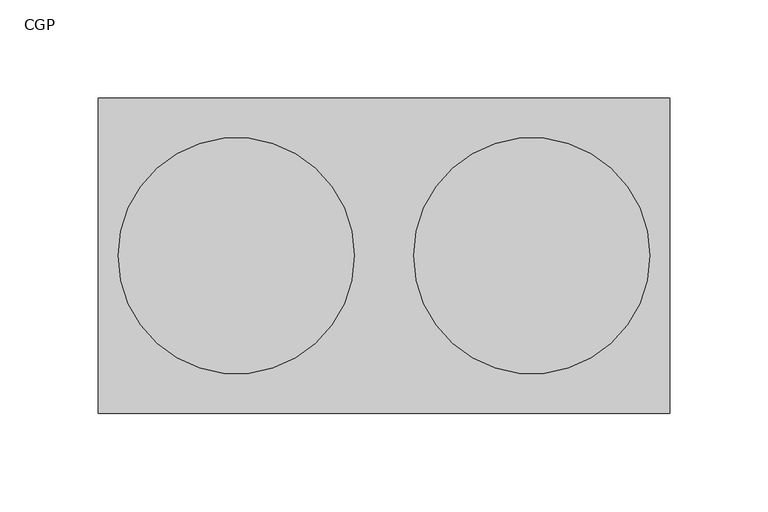
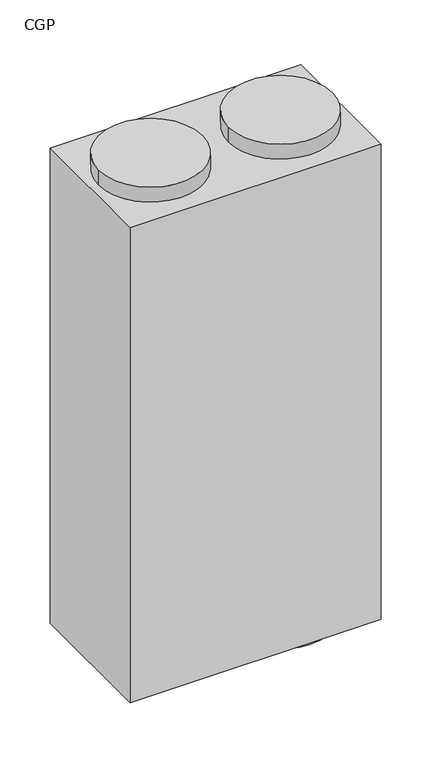
"""IFC4 building model written with IfcOpenShell, lengths in millimetres: proxy geometry, ELE-CGP : CGP."""

from ifc_helpers import new_model, si_unit, point, frame, frame_2d, origin, place, context, project, spatial, polyline, circle_curve, trimmed, segment, composite_curve, outline, extrude, source, transform, mapped, element, save


def cgp_80b3b499(model_context):
    return source(origin(), model_context, "Body", "SweptSolid", [
        extrude(outline(composite_curve([segment(trimmed(circle_curve(frame_2d((-75.0, -80.0)), 60.0), [point((-15.0, -80.0))], [point((-135.0, -80.0))], False, "CARTESIAN"), True, "CONTINUOUS"), segment(trimmed(circle_curve(frame_2d((-75.0, -80.0)), 60.0), [point((-135.0, -80.0))], [point((-15.0, -80.0))], False, "CARTESIAN"), True, "CONTINUOUS")], self_intersect=False)), frame((0.0, 0.0, 1580.0), z_axis=(0.0, 0.0, 1.0), x_axis=(1.0, 0.0, 0.0)), (0.0, 0.0, 1.0), 18.2289723),
        extrude(outline(composite_curve([segment(trimmed(circle_curve(frame_2d((75.0, -80.0)), 60.0), [point((15.0, -80.0))], [point((135.0, -80.0))], False, "CARTESIAN"), True, "CONTINUOUS"), segment(trimmed(circle_curve(frame_2d((75.0, -80.0)), 60.0), [point((135.0, -80.0))], [point((15.0, -80.0))], False, "CARTESIAN"), True, "CONTINUOUS")], self_intersect=False)), frame((0.0, 0.0, 1580.0), z_axis=(0.0, 0.0, 1.0), x_axis=(1.0, 0.0, 0.0)), (0.0, 0.0, 1.0), 18.2289723),
        extrude(outline(composite_curve([segment(trimmed(circle_curve(frame_2d((75.0, -80.0)), 60.0), [point((15.0, -80.0))], [point((135.0, -80.0))], False, "CARTESIAN"), True, "CONTINUOUS"), segment(trimmed(circle_curve(frame_2d((75.0, -80.0)), 60.0), [point((135.0, -80.0))], [point((15.0, -80.0))], False, "CARTESIAN"), True, "CONTINUOUS")], self_intersect=False)), frame((0.0, 0.0, 981.7710277), z_axis=(0.0, 0.0, 1.0), x_axis=(1.0, 0.0, 0.0)), (0.0, 0.0, 1.0), 18.2289723),
        extrude(outline(polyline([(145.0, 0.0), (145.0, -160.0), (-145.0, -160.0), (-145.0, 0.0), (145.0, 0.0)])), frame((0.0, 0.0, 1000.0), z_axis=(0.0, 0.0, 1.0), x_axis=(1.0, 0.0, 0.0)), (0.0, 0.0, 1.0), 580.0),
    ])


if __name__ == "__main__":
    model = new_model("IFC4")
    model_context = context("Model", 3, world=origin())
    ifc_project = project(units=[si_unit("LENGTHUNIT", "METRE", prefix="MILLI")], contexts=[model_context])
    site = spatial("IfcSite", under=ifc_project)
    building = spatial("IfcBuilding", under=site)
    placement = place(None, origin())
    cgp_shape = cgp_80b3b499(model_context)
    element("IfcBuildingElementProxy", 1, Name="ELE-CGP : CGP", ObjectType="ELE-CGP : CGP", at=placement, inside=building, context=model_context, shape_type="MappedRepresentation", body=[
        mapped(cgp_shape, transform((0.0, 0.0, 0.0), x_axis=(1.0, 0.0, 0.0), y_axis=(0.0, 1.0, 0.0), z_axis=(0.0, 0.0, 1.0))),
    ])
    save(model, "model.ifc")

# Revit data of these elements
# Type "ELE-CGP : CGP"
#   Voltage = "380"
#   Profundidad = 0.16 m
#   built-in parameter 1140140 [instance default] = 1 (stored number, unit not read)
#   Elevación = 1.00 m
#   Diametro [instance default] = 0.16 m
#   Anchura = 0.29 m
#   Altura = 0.58 m
#   built-in parameter 1140142 [instance default] = -1
#   built-in parameter 1155100 [instance default] = -1
#   Default Elevation = 0
